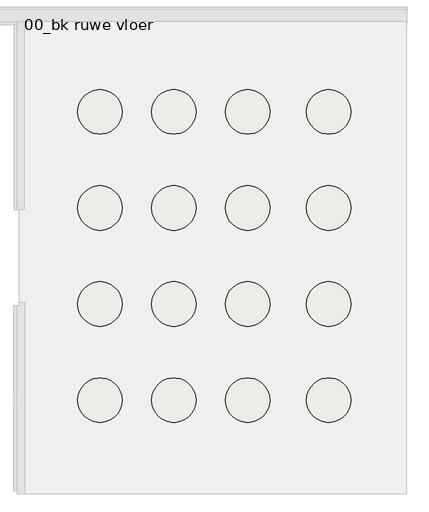
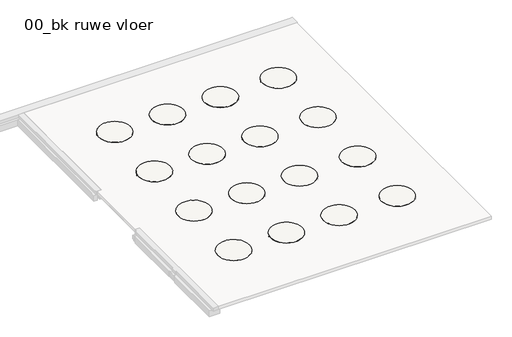
# One storey, part 3 of 6: 1 slab.
"""IFC4 building model written with IfcOpenShell, lengths in millimetres."""

from ifc_helpers import new_model, si_unit, frame, origin, place, context, project, spatial, circle_curve, element, save
from ifc_brep_helpers import plane_surface, cylinder_surface, advanced_brep

model = new_model("IFC4")

# Units and contexts
model_context = context("Model", 3, world=origin())
ifc_project = project(units=[si_unit("LENGTHUNIT", "METRE", prefix="MILLI")], contexts=[model_context])

# Site, building, storey
site = spatial("IfcSite", under=ifc_project)
building = spatial("IfcBuilding", under=site)
storey = spatial("IfcBuildingStorey", under=building, Name="00_bk ruwe vloer", Elevation=-70.0)

# Slab
placement = place(None, origin())
element("IfcSlab", 1, ObjectType="NLRS_23_FL_beton ihwg 450_gen_rsf", at=placement, inside=storey, context=model_context, shape_type="AdvancedBrep", body=[
    advanced_brep(
    [(34850.0, 37000.0, -520.0), (37850.0, 37000.0, -520.0), (37850.0, 37000.0, -70.0), (34850.0, 37000.0, -70.0), (34850.0, 37000.0, -390.0), (37850.0, 37000.0, -390.0), (37850.0, 37000.0, -330.0), (34850.0, 37000.0, -330.0), (37825.0, 37000.0, -390.0), (34875.0, 37000.0, -390.0), (37825.0, 37000.0, -330.0), (34875.0, 37000.0, -330.0)],
    [
        (0, 1, circle_curve(frame((36350.0, 37000.0, -520.0), z_axis=(0.0, 0.0, -1.0), x_axis=(1.0, 0.0, 0.0)), 1500.0)),
        (1, 0, circle_curve(frame((36350.0, 37000.0, -520.0), z_axis=(0.0, 0.0, -1.0), x_axis=(1.0, 0.0, 0.0)), 1500.0)),
        (2, 3, circle_curve(frame((36350.0, 37000.0, -70.0), z_axis=(0.0, 0.0, 1.0), x_axis=(1.0, 0.0, 0.0)), 1500.0)),
        (3, 2, circle_curve(frame((36350.0, 37000.0, -70.0), z_axis=(0.0, 0.0, 1.0), x_axis=(1.0, 0.0, 0.0)), 1500.0)),
        (0, 4),
        (4, 5, circle_curve(frame((36350.0, 37000.0, -390.0), z_axis=(0.0, 0.0, -1.0), x_axis=(1.0, 0.0, 0.0)), 1500.0)),
        (5, 1),
        (2, 6),
        (6, 7, circle_curve(frame((36350.0, 37000.0, -330.0), z_axis=(0.0, 0.0, 1.0), x_axis=(1.0, 0.0, 0.0)), 1500.0)),
        (7, 3),
        (5, 4, circle_curve(frame((36350.0, 37000.0, -390.0), z_axis=(0.0, 0.0, -1.0), x_axis=(1.0, 0.0, 0.0)), 1500.0)),
        (7, 6, circle_curve(frame((36350.0, 37000.0, -330.0), z_axis=(0.0, 0.0, 1.0), x_axis=(1.0, 0.0, 0.0)), 1500.0)),
        (8, 9, circle_curve(frame((36350.0, 37000.0, -390.0), z_axis=(0.0, 0.0, -1.0), x_axis=(1.0, 0.0, 0.0)), 1475.0)),
        (9, 8, circle_curve(frame((36350.0, 37000.0, -390.0), z_axis=(0.0, 0.0, -1.0), x_axis=(1.0, 0.0, 0.0)), 1475.0)),
        (10, 11, circle_curve(frame((36350.0, 37000.0, -330.0), z_axis=(0.0, 0.0, 1.0), x_axis=(1.0, 0.0, 0.0)), 1475.0)),
        (11, 10, circle_curve(frame((36350.0, 37000.0, -330.0), z_axis=(0.0, 0.0, 1.0), x_axis=(1.0, 0.0, 0.0)), 1475.0)),
        (8, 10),
        (11, 9),
    ],
    [
        plane_surface(frame((37850.0, 37000.0, -520.0), z_axis=(0.0, 0.0, -1.0), x_axis=(0.0, -1.0, 0.0))),
        plane_surface(frame((37850.0, 37000.0, -70.0), z_axis=(0.0, 0.0, 1.0), x_axis=(0.0, 1.0, 0.0))),
        cylinder_surface(frame((36350.0, 37000.0, -70.0), z_axis=(0.0, 0.0, -1.0), x_axis=(1.0, 0.0, 0.0)), 1500.0),
        plane_surface(frame((51875.0, 42925.0, -390.0), z_axis=(0.0, 0.0, 1.0), x_axis=(1.0, 0.0, 0.0))),
        plane_surface(frame((51875.0, 42925.0, -330.0), z_axis=(0.0, 0.0, -1.0), x_axis=(-1.0, 0.0, 0.0))),
        cylinder_surface(frame((36350.0, 37000.0, -70.0), z_axis=(0.0, 0.0, 1.0), x_axis=(1.0, 0.0, 0.0)), 1475.0),
    ],
    [
        (0, [[1, 2]]),
        (1, [[3, 4]]),
        (2, [[-1, 5, 6, 7]]),
        (2, [[-3, 8, 9, 10]]),
        (2, [[-2, -7, 11, -5]]),
        (2, [[-4, -10, 12, -8]]),
        (3, [[-6, -11], [13, 14]]),
        (4, [[-9, -12], [15, 16]]),
        (5, [[-13, 17, -16, 18]]),
        (5, [[-14, -18, -15, -17]]),
    ],
),
    advanced_brep(
    [(45350.0, 37000.0, -520.0), (48350.0, 37000.0, -520.0), (48350.0, 37000.0, -70.0), (45350.0, 37000.0, -70.0), (45350.0, 37000.0, -390.0), (48350.0, 37000.0, -390.0), (48350.0, 37000.0, -330.0), (45350.0, 37000.0, -330.0), (48325.0, 37000.0, -390.0), (45375.0, 37000.0, -390.0), (48325.0, 37000.0, -330.0), (45375.0, 37000.0, -330.0)],
    [
        (0, 1, circle_curve(frame((46850.0, 37000.0, -520.0), z_axis=(0.0, 0.0, -1.0), x_axis=(1.0, 0.0, 0.0)), 1500.0)),
        (1, 0, circle_curve(frame((46850.0, 37000.0, -520.0), z_axis=(0.0, 0.0, -1.0), x_axis=(1.0, 0.0, 0.0)), 1500.0)),
        (2, 3, circle_curve(frame((46850.0, 37000.0, -70.0), z_axis=(0.0, 0.0, 1.0), x_axis=(1.0, 0.0, 0.0)), 1500.0)),
        (3, 2, circle_curve(frame((46850.0, 37000.0, -70.0), z_axis=(0.0, 0.0, 1.0), x_axis=(1.0, 0.0, 0.0)), 1500.0)),
        (0, 4),
        (4, 5, circle_curve(frame((46850.0, 37000.0, -390.0), z_axis=(0.0, 0.0, -1.0), x_axis=(1.0, 0.0, 0.0)), 1500.0)),
        (5, 1),
        (2, 6),
        (6, 7, circle_curve(frame((46850.0, 37000.0, -330.0), z_axis=(0.0, 0.0, 1.0), x_axis=(1.0, 0.0, 0.0)), 1500.0)),
        (7, 3),
        (5, 4, circle_curve(frame((46850.0, 37000.0, -390.0), z_axis=(0.0, 0.0, -1.0), x_axis=(1.0, 0.0, 0.0)), 1500.0)),
        (7, 6, circle_curve(frame((46850.0, 37000.0, -330.0), z_axis=(0.0, 0.0, 1.0), x_axis=(1.0, 0.0, 0.0)), 1500.0)),
        (8, 9, circle_curve(frame((46850.0, 37000.0, -390.0), z_axis=(0.0, 0.0, -1.0), x_axis=(1.0, 0.0, 0.0)), 1475.0)),
        (9, 8, circle_curve(frame((46850.0, 37000.0, -390.0), z_axis=(0.0, 0.0, -1.0), x_axis=(1.0, 0.0, 0.0)), 1475.0)),
        (10, 11, circle_curve(frame((46850.0, 37000.0, -330.0), z_axis=(0.0, 0.0, 1.0), x_axis=(1.0, 0.0, 0.0)), 1475.0)),
        (11, 10, circle_curve(frame((46850.0, 37000.0, -330.0), z_axis=(0.0, 0.0, 1.0), x_axis=(1.0, 0.0, 0.0)), 1475.0)),
        (8, 10),
        (11, 9),
    ],
    [
        plane_surface(frame((37850.0, 37000.0, -520.0), z_axis=(0.0, 0.0, -1.0), x_axis=(0.0, -1.0, 0.0))),
        plane_surface(frame((37850.0, 37000.0, -70.0), z_axis=(0.0, 0.0, 1.0), x_axis=(0.0, 1.0, 0.0))),
        cylinder_surface(frame((46850.0, 37000.0, -70.0), z_axis=(0.0, 0.0, -1.0), x_axis=(1.0, 0.0, 0.0)), 1500.0),
        plane_surface(frame((51875.0, 42925.0, -390.0), z_axis=(0.0, 0.0, 1.0), x_axis=(1.0, 0.0, 0.0))),
        plane_surface(frame((51875.0, 42925.0, -330.0), z_axis=(0.0, 0.0, -1.0), x_axis=(-1.0, 0.0, 0.0))),
        cylinder_surface(frame((46850.0, 37000.0, -70.0), z_axis=(0.0, 0.0, 1.0), x_axis=(1.0, 0.0, 0.0)), 1475.0),
    ],
    [
        (0, [[1, 2]]),
        (1, [[3, 4]]),
        (2, [[-1, 5, 6, 7]]),
        (2, [[-3, 8, 9, 10]]),
        (2, [[-2, -7, 11, -5]]),
        (2, [[-4, -10, 12, -8]]),
        (3, [[-6, -11], [13, 14]]),
        (4, [[-9, -12], [15, 16]]),
        (5, [[-13, 17, -16, 18]]),
        (5, [[-14, -18, -15, -17]]),
    ],
),
    advanced_brep(
    [(45350.0, 30500.0, -520.0), (48350.0, 30500.0, -520.0), (48350.0, 30500.0, -70.0), (45350.0, 30500.0, -70.0), (45350.0, 30500.0, -390.0), (48350.0, 30500.0, -390.0), (48350.0, 30500.0, -330.0), (45350.0, 30500.0, -330.0), (48325.0, 30500.0, -390.0), (45375.0, 30500.0, -390.0), (48325.0, 30500.0, -330.0), (45375.0, 30500.0, -330.0)],
    [
        (0, 1, circle_curve(frame((46850.0, 30500.0, -520.0), z_axis=(0.0, 0.0, -1.0), x_axis=(1.0, 0.0, 0.0)), 1500.0)),
        (1, 0, circle_curve(frame((46850.0, 30500.0, -520.0), z_axis=(0.0, 0.0, -1.0), x_axis=(1.0, 0.0, 0.0)), 1500.0)),
        (2, 3, circle_curve(frame((46850.0, 30500.0, -70.0), z_axis=(0.0, 0.0, 1.0), x_axis=(1.0, 0.0, 0.0)), 1500.0)),
        (3, 2, circle_curve(frame((46850.0, 30500.0, -70.0), z_axis=(0.0, 0.0, 1.0), x_axis=(1.0, 0.0, 0.0)), 1500.0)),
        (0, 4),
        (4, 5, circle_curve(frame((46850.0, 30500.0, -390.0), z_axis=(0.0, 0.0, -1.0), x_axis=(1.0, 0.0, 0.0)), 1500.0)),
        (5, 1),
        (2, 6),
        (6, 7, circle_curve(frame((46850.0, 30500.0, -330.0), z_axis=(0.0, 0.0, 1.0), x_axis=(1.0, 0.0, 0.0)), 1500.0)),
        (7, 3),
        (5, 4, circle_curve(frame((46850.0, 30500.0, -390.0), z_axis=(0.0, 0.0, -1.0), x_axis=(1.0, 0.0, 0.0)), 1500.0)),
        (7, 6, circle_curve(frame((46850.0, 30500.0, -330.0), z_axis=(0.0, 0.0, 1.0), x_axis=(1.0, 0.0, 0.0)), 1500.0)),
        (8, 9, circle_curve(frame((46850.0, 30500.0, -390.0), z_axis=(0.0, 0.0, -1.0), x_axis=(1.0, 0.0, 0.0)), 1475.0)),
        (9, 8, circle_curve(frame((46850.0, 30500.0, -390.0), z_axis=(0.0, 0.0, -1.0), x_axis=(1.0, 0.0, 0.0)), 1475.0)),
        (10, 11, circle_curve(frame((46850.0, 30500.0, -330.0), z_axis=(0.0, 0.0, 1.0), x_axis=(1.0, 0.0, 0.0)), 1475.0)),
        (11, 10, circle_curve(frame((46850.0, 30500.0, -330.0), z_axis=(0.0, 0.0, 1.0), x_axis=(1.0, 0.0, 0.0)), 1475.0)),
        (8, 10),
        (11, 9),
    ],
    [
        plane_surface(frame((37850.0, 37000.0, -520.0), z_axis=(0.0, 0.0, -1.0), x_axis=(0.0, -1.0, 0.0))),
        plane_surface(frame((37850.0, 37000.0, -70.0), z_axis=(0.0, 0.0, 1.0), x_axis=(0.0, 1.0, 0.0))),
        cylinder_surface(frame((46850.0, 30500.0, -70.0), z_axis=(0.0, 0.0, -1.0), x_axis=(1.0, 0.0, 0.0)), 1500.0),
        plane_surface(frame((51875.0, 42925.0, -390.0), z_axis=(0.0, 0.0, 1.0), x_axis=(1.0, 0.0, 0.0))),
        plane_surface(frame((51875.0, 42925.0, -330.0), z_axis=(0.0, 0.0, -1.0), x_axis=(-1.0, 0.0, 0.0))),
        cylinder_surface(frame((46850.0, 30500.0, -70.0), z_axis=(0.0, 0.0, 1.0), x_axis=(1.0, 0.0, 0.0)), 1475.0),
    ],
    [
        (0, [[1, 2]]),
        (1, [[3, 4]]),
        (2, [[-1, 5, 6, 7]]),
        (2, [[-3, 8, 9, 10]]),
        (2, [[-2, -7, 11, -5]]),
        (2, [[-4, -10, 12, -8]]),
        (3, [[-6, -11], [13, 14]]),
        (4, [[-9, -12], [15, 16]]),
        (5, [[-13, 17, -16, 18]]),
        (5, [[-14, -18, -15, -17]]),
    ],
),
    advanced_brep(
    [(34850.0, 30500.0, -520.0), (37850.0, 30500.0, -520.0), (37850.0, 30500.0, -70.0), (34850.0, 30500.0, -70.0), (34850.0, 30500.0, -390.0), (37850.0, 30500.0, -390.0), (37850.0, 30500.0, -330.0), (34850.0, 30500.0, -330.0), (37825.0, 30500.0, -390.0), (34875.0, 30500.0, -390.0), (37825.0, 30500.0, -330.0), (34875.0, 30500.0, -330.0)],
    [
        (0, 1, circle_curve(frame((36350.0, 30500.0, -520.0), z_axis=(0.0, 0.0, -1.0), x_axis=(1.0, 0.0, 0.0)), 1500.0)),
        (1, 0, circle_curve(frame((36350.0, 30500.0, -520.0), z_axis=(0.0, 0.0, -1.0), x_axis=(1.0, 0.0, 0.0)), 1500.0)),
        (2, 3, circle_curve(frame((36350.0, 30500.0, -70.0), z_axis=(0.0, 0.0, 1.0), x_axis=(1.0, 0.0, 0.0)), 1500.0)),
        (3, 2, circle_curve(frame((36350.0, 30500.0, -70.0), z_axis=(0.0, 0.0, 1.0), x_axis=(1.0, 0.0, 0.0)), 1500.0)),
        (0, 4),
        (4, 5, circle_curve(frame((36350.0, 30500.0, -390.0), z_axis=(0.0, 0.0, -1.0), x_axis=(1.0, 0.0, 0.0)), 1500.0)),
        (5, 1),
        (2, 6),
        (6, 7, circle_curve(frame((36350.0, 30500.0, -330.0), z_axis=(0.0, 0.0, 1.0), x_axis=(1.0, 0.0, 0.0)), 1500.0)),
        (7, 3),
        (5, 4, circle_curve(frame((36350.0, 30500.0, -390.0), z_axis=(0.0, 0.0, -1.0), x_axis=(1.0, 0.0, 0.0)), 1500.0)),
        (7, 6, circle_curve(frame((36350.0, 30500.0, -330.0), z_axis=(0.0, 0.0, 1.0), x_axis=(1.0, 0.0, 0.0)), 1500.0)),
        (8, 9, circle_curve(frame((36350.0, 30500.0, -390.0), z_axis=(0.0, 0.0, -1.0), x_axis=(1.0, 0.0, 0.0)), 1475.0)),
        (9, 8, circle_curve(frame((36350.0, 30500.0, -390.0), z_axis=(0.0, 0.0, -1.0), x_axis=(1.0, 0.0, 0.0)), 1475.0)),
        (10, 11, circle_curve(frame((36350.0, 30500.0, -330.0), z_axis=(0.0, 0.0, 1.0), x_axis=(1.0, 0.0, 0.0)), 1475.0)),
        (11, 10, circle_curve(frame((36350.0, 30500.0, -330.0), z_axis=(0.0, 0.0, 1.0), x_axis=(1.0, 0.0, 0.0)), 1475.0)),
        (8, 10),
        (11, 9),
    ],
    [
        plane_surface(frame((37850.0, 37000.0, -520.0), z_axis=(0.0, 0.0, -1.0), x_axis=(0.0, -1.0, 0.0))),
        plane_surface(frame((37850.0, 37000.0, -70.0), z_axis=(0.0, 0.0, 1.0), x_axis=(0.0, 1.0, 0.0))),
        cylinder_surface(frame((36350.0, 30500.0, -70.0), z_axis=(0.0, 0.0, -1.0), x_axis=(1.0, 0.0, 0.0)), 1500.0),
        plane_surface(frame((51875.0, 42925.0, -390.0), z_axis=(0.0, 0.0, 1.0), x_axis=(1.0, 0.0, 0.0))),
        plane_surface(frame((51875.0, 42925.0, -330.0), z_axis=(0.0, 0.0, -1.0), x_axis=(-1.0, 0.0, 0.0))),
        cylinder_surface(frame((36350.0, 30500.0, -70.0), z_axis=(0.0, 0.0, 1.0), x_axis=(1.0, 0.0, 0.0)), 1475.0),
    ],
    [
        (0, [[1, 2]]),
        (1, [[3, 4]]),
        (2, [[-1, 5, 6, 7]]),
        (2, [[-3, 8, 9, 10]]),
        (2, [[-2, -7, 11, -5]]),
        (2, [[-4, -10, 12, -8]]),
        (3, [[-6, -11], [13, 14]]),
        (4, [[-9, -12], [15, 16]]),
        (5, [[-13, 17, -16, 18]]),
        (5, [[-14, -18, -15, -17]]),
    ],
),
    advanced_brep(
    [(34850.0, 24000.0, -520.0), (37850.0, 24000.0, -520.0), (37850.0, 24000.0, -70.0), (34850.0, 24000.0, -70.0), (34850.0, 24000.0, -390.0), (37850.0, 24000.0, -390.0), (37850.0, 24000.0, -330.0), (34850.0, 24000.0, -330.0), (37825.0, 24000.0, -390.0), (34875.0, 24000.0, -390.0), (37825.0, 24000.0, -330.0), (34875.0, 24000.0, -330.0)],
    [
        (0, 1, circle_curve(frame((36350.0, 24000.0, -520.0), z_axis=(0.0, 0.0, -1.0), x_axis=(1.0, 0.0, 0.0)), 1500.0)),
        (1, 0, circle_curve(frame((36350.0, 24000.0, -520.0), z_axis=(0.0, 0.0, -1.0), x_axis=(1.0, 0.0, 0.0)), 1500.0)),
        (2, 3, circle_curve(frame((36350.0, 24000.0, -70.0), z_axis=(0.0, 0.0, 1.0), x_axis=(1.0, 0.0, 0.0)), 1500.0)),
        (3, 2, circle_curve(frame((36350.0, 24000.0, -70.0), z_axis=(0.0, 0.0, 1.0), x_axis=(1.0, 0.0, 0.0)), 1500.0)),
        (0, 4),
        (4, 5, circle_curve(frame((36350.0, 24000.0, -390.0), z_axis=(0.0, 0.0, -1.0), x_axis=(1.0, 0.0, 0.0)), 1500.0)),
        (5, 1),
        (2, 6),
        (6, 7, circle_curve(frame((36350.0, 24000.0, -330.0), z_axis=(0.0, 0.0, 1.0), x_axis=(1.0, 0.0, 0.0)), 1500.0)),
        (7, 3),
        (5, 4, circle_curve(frame((36350.0, 24000.0, -390.0), z_axis=(0.0, 0.0, -1.0), x_axis=(1.0, 0.0, 0.0)), 1500.0)),
        (7, 6, circle_curve(frame((36350.0, 24000.0, -330.0), z_axis=(0.0, 0.0, 1.0), x_axis=(1.0, 0.0, 0.0)), 1500.0)),
        (8, 9, circle_curve(frame((36350.0, 24000.0, -390.0), z_axis=(0.0, 0.0, -1.0), x_axis=(1.0, 0.0, 0.0)), 1475.0)),
        (9, 8, circle_curve(frame((36350.0, 24000.0, -390.0), z_axis=(0.0, 0.0, -1.0), x_axis=(1.0, 0.0, 0.0)), 1475.0)),
        (10, 11, circle_curve(frame((36350.0, 24000.0, -330.0), z_axis=(0.0, 0.0, 1.0), x_axis=(1.0, 0.0, 0.0)), 1475.0)),
        (11, 10, circle_curve(frame((36350.0, 24000.0, -330.0), z_axis=(0.0, 0.0, 1.0), x_axis=(1.0, 0.0, 0.0)), 1475.0)),
        (8, 10),
        (11, 9),
    ],
    [
        plane_surface(frame((37850.0, 37000.0, -520.0), z_axis=(0.0, 0.0, -1.0), x_axis=(0.0, -1.0, 0.0))),
        plane_surface(frame((37850.0, 37000.0, -70.0), z_axis=(0.0, 0.0, 1.0), x_axis=(0.0, 1.0, 0.0))),
        cylinder_surface(frame((36350.0, 24000.0, -70.0), z_axis=(0.0, 0.0, -1.0), x_axis=(1.0, 0.0, 0.0)), 1500.0),
        plane_surface(frame((51875.0, 42925.0, -390.0), z_axis=(0.0, 0.0, 1.0), x_axis=(1.0, 0.0, 0.0))),
        plane_surface(frame((51875.0, 42925.0, -330.0), z_axis=(0.0, 0.0, -1.0), x_axis=(-1.0, 0.0, 0.0))),
        cylinder_surface(frame((36350.0, 24000.0, -70.0), z_axis=(0.0, 0.0, 1.0), x_axis=(1.0, 0.0, 0.0)), 1475.0),
    ],
    [
        (0, [[1, 2]]),
        (1, [[3, 4]]),
        (2, [[-1, 5, 6, 7]]),
        (2, [[-3, 8, 9, 10]]),
        (2, [[-2, -7, 11, -5]]),
        (2, [[-4, -10, 12, -8]]),
        (3, [[-6, -11], [13, 14]]),
        (4, [[-9, -12], [15, 16]]),
        (5, [[-13, 17, -16, 18]]),
        (5, [[-14, -18, -15, -17]]),
    ],
),
    advanced_brep(
    [(45350.0, 24000.0, -520.0), (48350.0, 24000.0, -520.0), (48350.0, 24000.0, -70.0), (45350.0, 24000.0, -70.0), (45350.0, 24000.0, -390.0), (48350.0, 24000.0, -390.0), (48350.0, 24000.0, -330.0), (45350.0, 24000.0, -330.0), (48325.0, 24000.0, -390.0), (45375.0, 24000.0, -390.0), (48325.0, 24000.0, -330.0), (45375.0, 24000.0, -330.0)],
    [
        (0, 1, circle_curve(frame((46850.0, 24000.0, -520.0), z_axis=(0.0, 0.0, -1.0), x_axis=(1.0, 0.0, 0.0)), 1500.0)),
        (1, 0, circle_curve(frame((46850.0, 24000.0, -520.0), z_axis=(0.0, 0.0, -1.0), x_axis=(1.0, 0.0, 0.0)), 1500.0)),
        (2, 3, circle_curve(frame((46850.0, 24000.0, -70.0), z_axis=(0.0, 0.0, 1.0), x_axis=(1.0, 0.0, 0.0)), 1500.0)),
        (3, 2, circle_curve(frame((46850.0, 24000.0, -70.0), z_axis=(0.0, 0.0, 1.0), x_axis=(1.0, 0.0, 0.0)), 1500.0)),
        (0, 4),
        (4, 5, circle_curve(frame((46850.0, 24000.0, -390.0), z_axis=(0.0, 0.0, -1.0), x_axis=(1.0, 0.0, 0.0)), 1500.0)),
        (5, 1),
        (2, 6),
        (6, 7, circle_curve(frame((46850.0, 24000.0, -330.0), z_axis=(0.0, 0.0, 1.0), x_axis=(1.0, 0.0, 0.0)), 1500.0)),
        (7, 3),
        (5, 4, circle_curve(frame((46850.0, 24000.0, -390.0), z_axis=(0.0, 0.0, -1.0), x_axis=(1.0, 0.0, 0.0)), 1500.0)),
        (7, 6, circle_curve(frame((46850.0, 24000.0, -330.0), z_axis=(0.0, 0.0, 1.0), x_axis=(1.0, 0.0, 0.0)), 1500.0)),
        (8, 9, circle_curve(frame((46850.0, 24000.0, -390.0), z_axis=(0.0, 0.0, -1.0), x_axis=(1.0, 0.0, 0.0)), 1475.0)),
        (9, 8, circle_curve(frame((46850.0, 24000.0, -390.0), z_axis=(0.0, 0.0, -1.0), x_axis=(1.0, 0.0, 0.0)), 1475.0)),
        (10, 11, circle_curve(frame((46850.0, 24000.0, -330.0), z_axis=(0.0, 0.0, 1.0), x_axis=(1.0, 0.0, 0.0)), 1475.0)),
        (11, 10, circle_curve(frame((46850.0, 24000.0, -330.0), z_axis=(0.0, 0.0, 1.0), x_axis=(1.0, 0.0, 0.0)), 1475.0)),
        (8, 10),
        (11, 9),
    ],
    [
        plane_surface(frame((37850.0, 37000.0, -520.0), z_axis=(0.0, 0.0, -1.0), x_axis=(0.0, -1.0, 0.0))),
        plane_surface(frame((37850.0, 37000.0, -70.0), z_axis=(0.0, 0.0, 1.0), x_axis=(0.0, 1.0, 0.0))),
        cylinder_surface(frame((46850.0, 24000.0, -70.0), z_axis=(0.0, 0.0, -1.0), x_axis=(1.0, 0.0, 0.0)), 1500.0),
        plane_surface(frame((51875.0, 42925.0, -390.0), z_axis=(0.0, 0.0, 1.0), x_axis=(1.0, 0.0, 0.0))),
        plane_surface(frame((51875.0, 42925.0, -330.0), z_axis=(0.0, 0.0, -1.0), x_axis=(-1.0, 0.0, 0.0))),
        cylinder_surface(frame((46850.0, 24000.0, -70.0), z_axis=(0.0, 0.0, 1.0), x_axis=(1.0, 0.0, 0.0)), 1475.0),
    ],
    [
        (0, [[1, 2]]),
        (1, [[3, 4]]),
        (2, [[-1, 5, 6, 7]]),
        (2, [[-3, 8, 9, 10]]),
        (2, [[-2, -7, 11, -5]]),
        (2, [[-4, -10, 12, -8]]),
        (3, [[-6, -11], [13, 14]]),
        (4, [[-9, -12], [15, 16]]),
        (5, [[-13, 17, -16, 18]]),
        (5, [[-14, -18, -15, -17]]),
    ],
),
    advanced_brep(
    [(45350.0, 17500.0, -520.0), (48350.0, 17500.0, -520.0), (48350.0, 17500.0, -70.0), (45350.0, 17500.0, -70.0), (45350.0, 17500.0, -390.0), (48350.0, 17500.0, -390.0), (48350.0, 17500.0, -330.0), (45350.0, 17500.0, -330.0), (48325.0, 17500.0, -390.0), (45375.0, 17500.0, -390.0), (48325.0, 17500.0, -330.0), (45375.0, 17500.0, -330.0)],
    [
        (0, 1, circle_curve(frame((46850.0, 17500.0, -520.0), z_axis=(0.0, 0.0, -1.0), x_axis=(1.0, 0.0, 0.0)), 1500.0)),
        (1, 0, circle_curve(frame((46850.0, 17500.0, -520.0), z_axis=(0.0, 0.0, -1.0), x_axis=(1.0, 0.0, 0.0)), 1500.0)),
        (2, 3, circle_curve(frame((46850.0, 17500.0, -70.0), z_axis=(0.0, 0.0, 1.0), x_axis=(1.0, 0.0, 0.0)), 1500.0)),
        (3, 2, circle_curve(frame((46850.0, 17500.0, -70.0), z_axis=(0.0, 0.0, 1.0), x_axis=(1.0, 0.0, 0.0)), 1500.0)),
        (0, 4),
        (4, 5, circle_curve(frame((46850.0, 17500.0, -390.0), z_axis=(0.0, 0.0, -1.0), x_axis=(1.0, 0.0, 0.0)), 1500.0)),
        (5, 1),
        (2, 6),
        (6, 7, circle_curve(frame((46850.0, 17500.0, -330.0), z_axis=(0.0, 0.0, 1.0), x_axis=(1.0, 0.0, 0.0)), 1500.0)),
        (7, 3),
        (5, 4, circle_curve(frame((46850.0, 17500.0, -390.0), z_axis=(0.0, 0.0, -1.0), x_axis=(1.0, 0.0, 0.0)), 1500.0)),
        (7, 6, circle_curve(frame((46850.0, 17500.0, -330.0), z_axis=(0.0, 0.0, 1.0), x_axis=(1.0, 0.0, 0.0)), 1500.0)),
        (8, 9, circle_curve(frame((46850.0, 17500.0, -390.0), z_axis=(0.0, 0.0, -1.0), x_axis=(1.0, 0.0, 0.0)), 1475.0)),
        (9, 8, circle_curve(frame((46850.0, 17500.0, -390.0), z_axis=(0.0, 0.0, -1.0), x_axis=(1.0, 0.0, 0.0)), 1475.0)),
        (10, 11, circle_curve(frame((46850.0, 17500.0, -330.0), z_axis=(0.0, 0.0, 1.0), x_axis=(1.0, 0.0, 0.0)), 1475.0)),
        (11, 10, circle_curve(frame((46850.0, 17500.0, -330.0), z_axis=(0.0, 0.0, 1.0), x_axis=(1.0, 0.0, 0.0)), 1475.0)),
        (8, 10),
        (11, 9),
    ],
    [
        plane_surface(frame((37850.0, 37000.0, -520.0), z_axis=(0.0, 0.0, -1.0), x_axis=(0.0, -1.0, 0.0))),
        plane_surface(frame((37850.0, 37000.0, -70.0), z_axis=(0.0, 0.0, 1.0), x_axis=(0.0, 1.0, 0.0))),
        cylinder_surface(frame((46850.0, 17500.0, -70.0), z_axis=(0.0, 0.0, -1.0), x_axis=(1.0, 0.0, 0.0)), 1500.0),
        plane_surface(frame((51875.0, 42925.0, -390.0), z_axis=(0.0, 0.0, 1.0), x_axis=(1.0, 0.0, 0.0))),
        plane_surface(frame((51875.0, 42925.0, -330.0), z_axis=(0.0, 0.0, -1.0), x_axis=(-1.0, 0.0, 0.0))),
        cylinder_surface(frame((46850.0, 17500.0, -70.0), z_axis=(0.0, 0.0, 1.0), x_axis=(1.0, 0.0, 0.0)), 1475.0),
    ],
    [
        (0, [[1, 2]]),
        (1, [[3, 4]]),
        (2, [[-1, 5, 6, 7]]),
        (2, [[-3, 8, 9, 10]]),
        (2, [[-2, -7, 11, -5]]),
        (2, [[-4, -10, 12, -8]]),
        (3, [[-6, -11], [13, 14]]),
        (4, [[-9, -12], [15, 16]]),
        (5, [[-13, 17, -16, 18]]),
        (5, [[-14, -18, -15, -17]]),
    ],
),
    advanced_brep(
    [(34850.0, 17500.0, -520.0), (37850.0, 17500.0, -520.0), (37850.0, 17500.0, -70.0), (34850.0, 17500.0, -70.0), (34850.0, 17500.0, -390.0), (37850.0, 17500.0, -390.0), (37850.0, 17500.0, -330.0), (34850.0, 17500.0, -330.0), (37825.0, 17500.0, -390.0), (34875.0, 17500.0, -390.0), (37825.0, 17500.0, -330.0), (34875.0, 17500.0, -330.0)],
    [
        (0, 1, circle_curve(frame((36350.0, 17500.0, -520.0), z_axis=(0.0, 0.0, -1.0), x_axis=(1.0, 0.0, 0.0)), 1500.0)),
        (1, 0, circle_curve(frame((36350.0, 17500.0, -520.0), z_axis=(0.0, 0.0, -1.0), x_axis=(1.0, 0.0, 0.0)), 1500.0)),
        (2, 3, circle_curve(frame((36350.0, 17500.0, -70.0), z_axis=(0.0, 0.0, 1.0), x_axis=(1.0, 0.0, 0.0)), 1500.0)),
        (3, 2, circle_curve(frame((36350.0, 17500.0, -70.0), z_axis=(0.0, 0.0, 1.0), x_axis=(1.0, 0.0, 0.0)), 1500.0)),
        (0, 4),
        (4, 5, circle_curve(frame((36350.0, 17500.0, -390.0), z_axis=(0.0, 0.0, -1.0), x_axis=(1.0, 0.0, 0.0)), 1500.0)),
        (5, 1),
        (2, 6),
        (6, 7, circle_curve(frame((36350.0, 17500.0, -330.0), z_axis=(0.0, 0.0, 1.0), x_axis=(1.0, 0.0, 0.0)), 1500.0)),
        (7, 3),
        (5, 4, circle_curve(frame((36350.0, 17500.0, -390.0), z_axis=(0.0, 0.0, -1.0), x_axis=(1.0, 0.0, 0.0)), 1500.0)),
        (7, 6, circle_curve(frame((36350.0, 17500.0, -330.0), z_axis=(0.0, 0.0, 1.0), x_axis=(1.0, 0.0, 0.0)), 1500.0)),
        (8, 9, circle_curve(frame((36350.0, 17500.0, -390.0), z_axis=(0.0, 0.0, -1.0), x_axis=(1.0, 0.0, 0.0)), 1475.0)),
        (9, 8, circle_curve(frame((36350.0, 17500.0, -390.0), z_axis=(0.0, 0.0, -1.0), x_axis=(1.0, 0.0, 0.0)), 1475.0)),
        (10, 11, circle_curve(frame((36350.0, 17500.0, -330.0), z_axis=(0.0, 0.0, 1.0), x_axis=(1.0, 0.0, 0.0)), 1475.0)),
        (11, 10, circle_curve(frame((36350.0, 17500.0, -330.0), z_axis=(0.0, 0.0, 1.0), x_axis=(1.0, 0.0, 0.0)), 1475.0)),
        (8, 10),
        (11, 9),
    ],
    [
        plane_surface(frame((37850.0, 37000.0, -520.0), z_axis=(0.0, 0.0, -1.0), x_axis=(0.0, -1.0, 0.0))),
        plane_surface(frame((37850.0, 37000.0, -70.0), z_axis=(0.0, 0.0, 1.0), x_axis=(0.0, 1.0, 0.0))),
        cylinder_surface(frame((36350.0, 17500.0, -70.0), z_axis=(0.0, 0.0, -1.0), x_axis=(1.0, 0.0, 0.0)), 1500.0),
        plane_surface(frame((51875.0, 42925.0, -390.0), z_axis=(0.0, 0.0, 1.0), x_axis=(1.0, 0.0, 0.0))),
        plane_surface(frame((51875.0, 42925.0, -330.0), z_axis=(0.0, 0.0, -1.0), x_axis=(-1.0, 0.0, 0.0))),
        cylinder_surface(frame((36350.0, 17500.0, -70.0), z_axis=(0.0, 0.0, 1.0), x_axis=(1.0, 0.0, 0.0)), 1475.0),
    ],
    [
        (0, [[1, 2]]),
        (1, [[3, 4]]),
        (2, [[-1, 5, 6, 7]]),
        (2, [[-3, 8, 9, 10]]),
        (2, [[-2, -7, 11, -5]]),
        (2, [[-4, -10, 12, -8]]),
        (3, [[-6, -11], [13, 14]]),
        (4, [[-9, -12], [15, 16]]),
        (5, [[-13, 17, -16, 18]]),
        (5, [[-14, -18, -15, -17]]),
    ],
),
    advanced_brep(
    [(39850.0, 37000.0, -520.0), (42850.0, 37000.0, -520.0), (42850.0, 37000.0, -70.0), (39850.0, 37000.0, -70.0), (39850.0, 37000.0, -390.0), (42850.0, 37000.0, -390.0), (42850.0, 37000.0, -330.0), (39850.0, 37000.0, -330.0), (42825.0, 37000.0, -390.0), (39875.0, 37000.0, -390.0), (42825.0, 37000.0, -330.0), (39875.0, 37000.0, -330.0)],
    [
        (0, 1, circle_curve(frame((41350.0, 37000.0, -520.0), z_axis=(0.0, 0.0, -1.0), x_axis=(1.0, 0.0, 0.0)), 1500.0)),
        (1, 0, circle_curve(frame((41350.0, 37000.0, -520.0), z_axis=(0.0, 0.0, -1.0), x_axis=(1.0, 0.0, 0.0)), 1500.0)),
        (2, 3, circle_curve(frame((41350.0, 37000.0, -70.0), z_axis=(0.0, 0.0, 1.0), x_axis=(1.0, 0.0, 0.0)), 1500.0)),
        (3, 2, circle_curve(frame((41350.0, 37000.0, -70.0), z_axis=(0.0, 0.0, 1.0), x_axis=(1.0, 0.0, 0.0)), 1500.0)),
        (0, 4),
        (4, 5, circle_curve(frame((41350.0, 37000.0, -390.0), z_axis=(0.0, 0.0, -1.0), x_axis=(1.0, 0.0, 0.0)), 1500.0)),
        (5, 1),
        (2, 6),
        (6, 7, circle_curve(frame((41350.0, 37000.0, -330.0), z_axis=(0.0, 0.0, 1.0), x_axis=(1.0, 0.0, 0.0)), 1500.0)),
        (7, 3),
        (5, 4, circle_curve(frame((41350.0, 37000.0, -390.0), z_axis=(0.0, 0.0, -1.0), x_axis=(1.0, 0.0, 0.0)), 1500.0)),
        (7, 6, circle_curve(frame((41350.0, 37000.0, -330.0), z_axis=(0.0, 0.0, 1.0), x_axis=(1.0, 0.0, 0.0)), 1500.0)),
        (8, 9, circle_curve(frame((41350.0, 37000.0, -390.0), z_axis=(0.0, 0.0, -1.0), x_axis=(1.0, 0.0, 0.0)), 1475.0)),
        (9, 8, circle_curve(frame((41350.0, 37000.0, -390.0), z_axis=(0.0, 0.0, -1.0), x_axis=(1.0, 0.0, 0.0)), 1475.0)),
        (10, 11, circle_curve(frame((41350.0, 37000.0, -330.0), z_axis=(0.0, 0.0, 1.0), x_axis=(1.0, 0.0, 0.0)), 1475.0)),
        (11, 10, circle_curve(frame((41350.0, 37000.0, -330.0), z_axis=(0.0, 0.0, 1.0), x_axis=(1.0, 0.0, 0.0)), 1475.0)),
        (8, 10),
        (11, 9),
    ],
    [
        plane_surface(frame((37850.0, 37000.0, -520.0), z_axis=(0.0, 0.0, -1.0), x_axis=(0.0, -1.0, 0.0))),
        plane_surface(frame((37850.0, 37000.0, -70.0), z_axis=(0.0, 0.0, 1.0), x_axis=(0.0, 1.0, 0.0))),
        cylinder_surface(frame((41350.0, 37000.0, -70.0), z_axis=(0.0, 0.0, -1.0), x_axis=(1.0, 0.0, 0.0)), 1500.0),
        plane_surface(frame((51875.0, 42925.0, -390.0), z_axis=(0.0, 0.0, 1.0), x_axis=(1.0, 0.0, 0.0))),
        plane_surface(frame((51875.0, 42925.0, -330.0), z_axis=(0.0, 0.0, -1.0), x_axis=(-1.0, 0.0, 0.0))),
        cylinder_surface(frame((41350.0, 37000.0, -70.0), z_axis=(0.0, 0.0, 1.0), x_axis=(1.0, 0.0, 0.0)), 1475.0),
    ],
    [
        (0, [[1, 2]]),
        (1, [[3, 4]]),
        (2, [[-1, 5, 6, 7]]),
        (2, [[-3, 8, 9, 10]]),
        (2, [[-2, -7, 11, -5]]),
        (2, [[-4, -10, 12, -8]]),
        (3, [[-6, -11], [13, 14]]),
        (4, [[-9, -12], [15, 16]]),
        (5, [[-13, 17, -16, 18]]),
        (5, [[-14, -18, -15, -17]]),
    ],
),
    advanced_brep(
    [(39850.0, 30500.0, -520.0), (42850.0, 30500.0, -520.0), (42850.0, 30500.0, -70.0), (39850.0, 30500.0, -70.0), (39850.0, 30500.0, -390.0), (42850.0, 30500.0, -390.0), (42850.0, 30500.0, -330.0), (39850.0, 30500.0, -330.0), (42825.0, 30500.0, -390.0), (39875.0, 30500.0, -390.0), (42825.0, 30500.0, -330.0), (39875.0, 30500.0, -330.0)],
    [
        (0, 1, circle_curve(frame((41350.0, 30500.0, -520.0), z_axis=(0.0, 0.0, -1.0), x_axis=(1.0, 0.0, 0.0)), 1500.0)),
        (1, 0, circle_curve(frame((41350.0, 30500.0, -520.0), z_axis=(0.0, 0.0, -1.0), x_axis=(1.0, 0.0, 0.0)), 1500.0)),
        (2, 3, circle_curve(frame((41350.0, 30500.0, -70.0), z_axis=(0.0, 0.0, 1.0), x_axis=(1.0, 0.0, 0.0)), 1500.0)),
        (3, 2, circle_curve(frame((41350.0, 30500.0, -70.0), z_axis=(0.0, 0.0, 1.0), x_axis=(1.0, 0.0, 0.0)), 1500.0)),
        (0, 4),
        (4, 5, circle_curve(frame((41350.0, 30500.0, -390.0), z_axis=(0.0, 0.0, -1.0), x_axis=(1.0, 0.0, 0.0)), 1500.0)),
        (5, 1),
        (2, 6),
        (6, 7, circle_curve(frame((41350.0, 30500.0, -330.0), z_axis=(0.0, 0.0, 1.0), x_axis=(1.0, 0.0, 0.0)), 1500.0)),
        (7, 3),
        (5, 4, circle_curve(frame((41350.0, 30500.0, -390.0), z_axis=(0.0, 0.0, -1.0), x_axis=(1.0, 0.0, 0.0)), 1500.0)),
        (7, 6, circle_curve(frame((41350.0, 30500.0, -330.0), z_axis=(0.0, 0.0, 1.0), x_axis=(1.0, 0.0, 0.0)), 1500.0)),
        (8, 9, circle_curve(frame((41350.0, 30500.0, -390.0), z_axis=(0.0, 0.0, -1.0), x_axis=(1.0, 0.0, 0.0)), 1475.0)),
        (9, 8, circle_curve(frame((41350.0, 30500.0, -390.0), z_axis=(0.0, 0.0, -1.0), x_axis=(1.0, 0.0, 0.0)), 1475.0)),
        (10, 11, circle_curve(frame((41350.0, 30500.0, -330.0), z_axis=(0.0, 0.0, 1.0), x_axis=(1.0, 0.0, 0.0)), 1475.0)),
        (11, 10, circle_curve(frame((41350.0, 30500.0, -330.0), z_axis=(0.0, 0.0, 1.0), x_axis=(1.0, 0.0, 0.0)), 1475.0)),
        (8, 10),
        (11, 9),
    ],
    [
        plane_surface(frame((37850.0, 37000.0, -520.0), z_axis=(0.0, 0.0, -1.0), x_axis=(0.0, -1.0, 0.0))),
        plane_surface(frame((37850.0, 37000.0, -70.0), z_axis=(0.0, 0.0, 1.0), x_axis=(0.0, 1.0, 0.0))),
        cylinder_surface(frame((41350.0, 30500.0, -70.0), z_axis=(0.0, 0.0, -1.0), x_axis=(1.0, 0.0, 0.0)), 1500.0),
        plane_surface(frame((51875.0, 42925.0, -390.0), z_axis=(0.0, 0.0, 1.0), x_axis=(1.0, 0.0, 0.0))),
        plane_surface(frame((51875.0, 42925.0, -330.0), z_axis=(0.0, 0.0, -1.0), x_axis=(-1.0, 0.0, 0.0))),
        cylinder_surface(frame((41350.0, 30500.0, -70.0), z_axis=(0.0, 0.0, 1.0), x_axis=(1.0, 0.0, 0.0)), 1475.0),
    ],
    [
        (0, [[1, 2]]),
        (1, [[3, 4]]),
        (2, [[-1, 5, 6, 7]]),
        (2, [[-3, 8, 9, 10]]),
        (2, [[-2, -7, 11, -5]]),
        (2, [[-4, -10, 12, -8]]),
        (3, [[-6, -11], [13, 14]]),
        (4, [[-9, -12], [15, 16]]),
        (5, [[-13, 17, -16, 18]]),
        (5, [[-14, -18, -15, -17]]),
    ],
),
    advanced_brep(
    [(39850.0, 24000.0, -520.0), (42850.0, 24000.0, -520.0), (42850.0, 24000.0, -70.0), (39850.0, 24000.0, -70.0), (39850.0, 24000.0, -390.0), (42850.0, 24000.0, -390.0), (42850.0, 24000.0, -330.0), (39850.0, 24000.0, -330.0), (42825.0, 24000.0, -390.0), (39875.0, 24000.0, -390.0), (42825.0, 24000.0, -330.0), (39875.0, 24000.0, -330.0)],
    [
        (0, 1, circle_curve(frame((41350.0, 24000.0, -520.0), z_axis=(0.0, 0.0, -1.0), x_axis=(1.0, 0.0, 0.0)), 1500.0)),
        (1, 0, circle_curve(frame((41350.0, 24000.0, -520.0), z_axis=(0.0, 0.0, -1.0), x_axis=(1.0, 0.0, 0.0)), 1500.0)),
        (2, 3, circle_curve(frame((41350.0, 24000.0, -70.0), z_axis=(0.0, 0.0, 1.0), x_axis=(1.0, 0.0, 0.0)), 1500.0)),
        (3, 2, circle_curve(frame((41350.0, 24000.0, -70.0), z_axis=(0.0, 0.0, 1.0), x_axis=(1.0, 0.0, 0.0)), 1500.0)),
        (0, 4),
        (4, 5, circle_curve(frame((41350.0, 24000.0, -390.0), z_axis=(0.0, 0.0, -1.0), x_axis=(1.0, 0.0, 0.0)), 1500.0)),
        (5, 1),
        (2, 6),
        (6, 7, circle_curve(frame((41350.0, 24000.0, -330.0), z_axis=(0.0, 0.0, 1.0), x_axis=(1.0, 0.0, 0.0)), 1500.0)),
        (7, 3),
        (5, 4, circle_curve(frame((41350.0, 24000.0, -390.0), z_axis=(0.0, 0.0, -1.0), x_axis=(1.0, 0.0, 0.0)), 1500.0)),
        (7, 6, circle_curve(frame((41350.0, 24000.0, -330.0), z_axis=(0.0, 0.0, 1.0), x_axis=(1.0, 0.0, 0.0)), 1500.0)),
        (8, 9, circle_curve(frame((41350.0, 24000.0, -390.0), z_axis=(0.0, 0.0, -1.0), x_axis=(1.0, 0.0, 0.0)), 1475.0)),
        (9, 8, circle_curve(frame((41350.0, 24000.0, -390.0), z_axis=(0.0, 0.0, -1.0), x_axis=(1.0, 0.0, 0.0)), 1475.0)),
        (10, 11, circle_curve(frame((41350.0, 24000.0, -330.0), z_axis=(0.0, 0.0, 1.0), x_axis=(1.0, 0.0, 0.0)), 1475.0)),
        (11, 10, circle_curve(frame((41350.0, 24000.0, -330.0), z_axis=(0.0, 0.0, 1.0), x_axis=(1.0, 0.0, 0.0)), 1475.0)),
        (8, 10),
        (11, 9),
    ],
    [
        plane_surface(frame((37850.0, 37000.0, -520.0), z_axis=(0.0, 0.0, -1.0), x_axis=(0.0, -1.0, 0.0))),
        plane_surface(frame((37850.0, 37000.0, -70.0), z_axis=(0.0, 0.0, 1.0), x_axis=(0.0, 1.0, 0.0))),
        cylinder_surface(frame((41350.0, 24000.0, -70.0), z_axis=(0.0, 0.0, -1.0), x_axis=(1.0, 0.0, 0.0)), 1500.0),
        plane_surface(frame((51875.0, 42925.0, -390.0), z_axis=(0.0, 0.0, 1.0), x_axis=(1.0, 0.0, 0.0))),
        plane_surface(frame((51875.0, 42925.0, -330.0), z_axis=(0.0, 0.0, -1.0), x_axis=(-1.0, 0.0, 0.0))),
        cylinder_surface(frame((41350.0, 24000.0, -70.0), z_axis=(0.0, 0.0, 1.0), x_axis=(1.0, 0.0, 0.0)), 1475.0),
    ],
    [
        (0, [[1, 2]]),
        (1, [[3, 4]]),
        (2, [[-1, 5, 6, 7]]),
        (2, [[-3, 8, 9, 10]]),
        (2, [[-2, -7, 11, -5]]),
        (2, [[-4, -10, 12, -8]]),
        (3, [[-6, -11], [13, 14]]),
        (4, [[-9, -12], [15, 16]]),
        (5, [[-13, 17, -16, 18]]),
        (5, [[-14, -18, -15, -17]]),
    ],
),
    advanced_brep(
    [(39850.0, 17500.0, -520.0), (42850.0, 17500.0, -520.0), (42850.0, 17500.0, -70.0), (39850.0, 17500.0, -70.0), (39850.0, 17500.0, -390.0), (42850.0, 17500.0, -390.0), (42850.0, 17500.0, -330.0), (39850.0, 17500.0, -330.0), (42825.0, 17500.0, -390.0), (39875.0, 17500.0, -390.0), (42825.0, 17500.0, -330.0), (39875.0, 17500.0, -330.0)],
    [
        (0, 1, circle_curve(frame((41350.0, 17500.0, -520.0), z_axis=(0.0, 0.0, -1.0), x_axis=(1.0, 0.0, 0.0)), 1500.0)),
        (1, 0, circle_curve(frame((41350.0, 17500.0, -520.0), z_axis=(0.0, 0.0, -1.0), x_axis=(1.0, 0.0, 0.0)), 1500.0)),
        (2, 3, circle_curve(frame((41350.0, 17500.0, -70.0), z_axis=(0.0, 0.0, 1.0), x_axis=(1.0, 0.0, 0.0)), 1500.0)),
        (3, 2, circle_curve(frame((41350.0, 17500.0, -70.0), z_axis=(0.0, 0.0, 1.0), x_axis=(1.0, 0.0, 0.0)), 1500.0)),
        (0, 4),
        (4, 5, circle_curve(frame((41350.0, 17500.0, -390.0), z_axis=(0.0, 0.0, -1.0), x_axis=(1.0, 0.0, 0.0)), 1500.0)),
        (5, 1),
        (2, 6),
        (6, 7, circle_curve(frame((41350.0, 17500.0, -330.0), z_axis=(0.0, 0.0, 1.0), x_axis=(1.0, 0.0, 0.0)), 1500.0)),
        (7, 3),
        (5, 4, circle_curve(frame((41350.0, 17500.0, -390.0), z_axis=(0.0, 0.0, -1.0), x_axis=(1.0, 0.0, 0.0)), 1500.0)),
        (7, 6, circle_curve(frame((41350.0, 17500.0, -330.0), z_axis=(0.0, 0.0, 1.0), x_axis=(1.0, 0.0, 0.0)), 1500.0)),
        (8, 9, circle_curve(frame((41350.0, 17500.0, -390.0), z_axis=(0.0, 0.0, -1.0), x_axis=(1.0, 0.0, 0.0)), 1475.0)),
        (9, 8, circle_curve(frame((41350.0, 17500.0, -390.0), z_axis=(0.0, 0.0, -1.0), x_axis=(1.0, 0.0, 0.0)), 1475.0)),
        (10, 11, circle_curve(frame((41350.0, 17500.0, -330.0), z_axis=(0.0, 0.0, 1.0), x_axis=(1.0, 0.0, 0.0)), 1475.0)),
        (11, 10, circle_curve(frame((41350.0, 17500.0, -330.0), z_axis=(0.0, 0.0, 1.0), x_axis=(1.0, 0.0, 0.0)), 1475.0)),
        (8, 10),
        (11, 9),
    ],
    [
        plane_surface(frame((37850.0, 37000.0, -520.0), z_axis=(0.0, 0.0, -1.0), x_axis=(0.0, -1.0, 0.0))),
        plane_surface(frame((37850.0, 37000.0, -70.0), z_axis=(0.0, 0.0, 1.0), x_axis=(0.0, 1.0, 0.0))),
        cylinder_surface(frame((41350.0, 17500.0, -70.0), z_axis=(0.0, 0.0, -1.0), x_axis=(1.0, 0.0, 0.0)), 1500.0),
        plane_surface(frame((51875.0, 42925.0, -390.0), z_axis=(0.0, 0.0, 1.0), x_axis=(1.0, 0.0, 0.0))),
        plane_surface(frame((51875.0, 42925.0, -330.0), z_axis=(0.0, 0.0, -1.0), x_axis=(-1.0, 0.0, 0.0))),
        cylinder_surface(frame((41350.0, 17500.0, -70.0), z_axis=(0.0, 0.0, 1.0), x_axis=(1.0, 0.0, 0.0)), 1475.0),
    ],
    [
        (0, [[1, 2]]),
        (1, [[3, 4]]),
        (2, [[-1, 5, 6, 7]]),
        (2, [[-3, 8, 9, 10]]),
        (2, [[-2, -7, 11, -5]]),
        (2, [[-4, -10, 12, -8]]),
        (3, [[-6, -11], [13, 14]]),
        (4, [[-9, -12], [15, 16]]),
        (5, [[-13, 17, -16, 18]]),
        (5, [[-14, -18, -15, -17]]),
    ],
),
    advanced_brep(
    [(29850.0, 37000.0, -520.0), (32850.0, 37000.0, -520.0), (32850.0, 37000.0, -70.0), (29850.0, 37000.0, -70.0), (29850.0, 37000.0, -390.0), (32850.0, 37000.0, -390.0), (32850.0, 37000.0, -330.0), (29850.0, 37000.0, -330.0), (32825.0, 37000.0, -390.0), (29875.0, 37000.0, -390.0), (32825.0, 37000.0, -330.0), (29875.0, 37000.0, -330.0)],
    [
        (0, 1, circle_curve(frame((31350.0, 37000.0, -520.0), z_axis=(0.0, 0.0, -1.0), x_axis=(1.0, 0.0, 0.0)), 1500.0)),
        (1, 0, circle_curve(frame((31350.0, 37000.0, -520.0), z_axis=(0.0, 0.0, -1.0), x_axis=(1.0, 0.0, 0.0)), 1500.0)),
        (2, 3, circle_curve(frame((31350.0, 37000.0, -70.0), z_axis=(0.0, 0.0, 1.0), x_axis=(1.0, 0.0, 0.0)), 1500.0)),
        (3, 2, circle_curve(frame((31350.0, 37000.0, -70.0), z_axis=(0.0, 0.0, 1.0), x_axis=(1.0, 0.0, 0.0)), 1500.0)),
        (0, 4),
        (4, 5, circle_curve(frame((31350.0, 37000.0, -390.0), z_axis=(0.0, 0.0, -1.0), x_axis=(1.0, 0.0, 0.0)), 1500.0)),
        (5, 1),
        (2, 6),
        (6, 7, circle_curve(frame((31350.0, 37000.0, -330.0), z_axis=(0.0, 0.0, 1.0), x_axis=(1.0, 0.0, 0.0)), 1500.0)),
        (7, 3),
        (5, 4, circle_curve(frame((31350.0, 37000.0, -390.0), z_axis=(0.0, 0.0, -1.0), x_axis=(1.0, 0.0, 0.0)), 1500.0)),
        (7, 6, circle_curve(frame((31350.0, 37000.0, -330.0), z_axis=(0.0, 0.0, 1.0), x_axis=(1.0, 0.0, 0.0)), 1500.0)),
        (8, 9, circle_curve(frame((31350.0, 37000.0, -390.0), z_axis=(0.0, 0.0, -1.0), x_axis=(1.0, 0.0, 0.0)), 1475.0)),
        (9, 8, circle_curve(frame((31350.0, 37000.0, -390.0), z_axis=(0.0, 0.0, -1.0), x_axis=(1.0, 0.0, 0.0)), 1475.0)),
        (10, 11, circle_curve(frame((31350.0, 37000.0, -330.0), z_axis=(0.0, 0.0, 1.0), x_axis=(1.0, 0.0, 0.0)), 1475.0)),
        (11, 10, circle_curve(frame((31350.0, 37000.0, -330.0), z_axis=(0.0, 0.0, 1.0), x_axis=(1.0, 0.0, 0.0)), 1475.0)),
        (8, 10),
        (11, 9),
    ],
    [
        plane_surface(frame((37850.0, 37000.0, -520.0), z_axis=(0.0, 0.0, -1.0), x_axis=(0.0, -1.0, 0.0))),
        plane_surface(frame((37850.0, 37000.0, -70.0), z_axis=(0.0, 0.0, 1.0), x_axis=(0.0, 1.0, 0.0))),
        cylinder_surface(frame((31350.0, 37000.0, -70.0), z_axis=(0.0, 0.0, -1.0), x_axis=(1.0, 0.0, 0.0)), 1500.0),
        plane_surface(frame((51875.0, 42925.0, -390.0), z_axis=(0.0, 0.0, 1.0), x_axis=(1.0, 0.0, 0.0))),
        plane_surface(frame((51875.0, 42925.0, -330.0), z_axis=(0.0, 0.0, -1.0), x_axis=(-1.0, 0.0, 0.0))),
        cylinder_surface(frame((31350.0, 37000.0, -70.0), z_axis=(0.0, 0.0, 1.0), x_axis=(1.0, 0.0, 0.0)), 1475.0),
    ],
    [
        (0, [[1, 2]]),
        (1, [[3, 4]]),
        (2, [[-1, 5, 6, 7]]),
        (2, [[-3, 8, 9, 10]]),
        (2, [[-2, -7, 11, -5]]),
        (2, [[-4, -10, 12, -8]]),
        (3, [[-6, -11], [13, 14]]),
        (4, [[-9, -12], [15, 16]]),
        (5, [[-13, 17, -16, 18]]),
        (5, [[-14, -18, -15, -17]]),
    ],
),
    advanced_brep(
    [(29850.0, 30500.0, -520.0), (32850.0, 30500.0, -520.0), (32850.0, 30500.0, -70.0), (29850.0, 30500.0, -70.0), (29850.0, 30500.0, -390.0), (32850.0, 30500.0, -390.0), (32850.0, 30500.0, -330.0), (29850.0, 30500.0, -330.0), (32825.0, 30500.0, -390.0), (29875.0, 30500.0, -390.0), (32825.0, 30500.0, -330.0), (29875.0, 30500.0, -330.0)],
    [
        (0, 1, circle_curve(frame((31350.0, 30500.0, -520.0), z_axis=(0.0, 0.0, -1.0), x_axis=(1.0, 0.0, 0.0)), 1500.0)),
        (1, 0, circle_curve(frame((31350.0, 30500.0, -520.0), z_axis=(0.0, 0.0, -1.0), x_axis=(1.0, 0.0, 0.0)), 1500.0)),
        (2, 3, circle_curve(frame((31350.0, 30500.0, -70.0), z_axis=(0.0, 0.0, 1.0), x_axis=(1.0, 0.0, 0.0)), 1500.0)),
        (3, 2, circle_curve(frame((31350.0, 30500.0, -70.0), z_axis=(0.0, 0.0, 1.0), x_axis=(1.0, 0.0, 0.0)), 1500.0)),
        (0, 4),
        (4, 5, circle_curve(frame((31350.0, 30500.0, -390.0), z_axis=(0.0, 0.0, -1.0), x_axis=(1.0, 0.0, 0.0)), 1500.0)),
        (5, 1),
        (2, 6),
        (6, 7, circle_curve(frame((31350.0, 30500.0, -330.0), z_axis=(0.0, 0.0, 1.0), x_axis=(1.0, 0.0, 0.0)), 1500.0)),
        (7, 3),
        (5, 4, circle_curve(frame((31350.0, 30500.0, -390.0), z_axis=(0.0, 0.0, -1.0), x_axis=(1.0, 0.0, 0.0)), 1500.0)),
        (7, 6, circle_curve(frame((31350.0, 30500.0, -330.0), z_axis=(0.0, 0.0, 1.0), x_axis=(1.0, 0.0, 0.0)), 1500.0)),
        (8, 9, circle_curve(frame((31350.0, 30500.0, -390.0), z_axis=(0.0, 0.0, -1.0), x_axis=(1.0, 0.0, 0.0)), 1475.0)),
        (9, 8, circle_curve(frame((31350.0, 30500.0, -390.0), z_axis=(0.0, 0.0, -1.0), x_axis=(1.0, 0.0, 0.0)), 1475.0)),
        (10, 11, circle_curve(frame((31350.0, 30500.0, -330.0), z_axis=(0.0, 0.0, 1.0), x_axis=(1.0, 0.0, 0.0)), 1475.0)),
        (11, 10, circle_curve(frame((31350.0, 30500.0, -330.0), z_axis=(0.0, 0.0, 1.0), x_axis=(1.0, 0.0, 0.0)), 1475.0)),
        (8, 10),
        (11, 9),
    ],
    [
        plane_surface(frame((37850.0, 37000.0, -520.0), z_axis=(0.0, 0.0, -1.0), x_axis=(0.0, -1.0, 0.0))),
        plane_surface(frame((37850.0, 37000.0, -70.0), z_axis=(0.0, 0.0, 1.0), x_axis=(0.0, 1.0, 0.0))),
        cylinder_surface(frame((31350.0, 30500.0, -70.0), z_axis=(0.0, 0.0, -1.0), x_axis=(1.0, 0.0, 0.0)), 1500.0),
        plane_surface(frame((51875.0, 42925.0, -390.0), z_axis=(0.0, 0.0, 1.0), x_axis=(1.0, 0.0, 0.0))),
        plane_surface(frame((51875.0, 42925.0, -330.0), z_axis=(0.0, 0.0, -1.0), x_axis=(-1.0, 0.0, 0.0))),
        cylinder_surface(frame((31350.0, 30500.0, -70.0), z_axis=(0.0, 0.0, 1.0), x_axis=(1.0, 0.0, 0.0)), 1475.0),
    ],
    [
        (0, [[1, 2]]),
        (1, [[3, 4]]),
        (2, [[-1, 5, 6, 7]]),
        (2, [[-3, 8, 9, 10]]),
        (2, [[-2, -7, 11, -5]]),
        (2, [[-4, -10, 12, -8]]),
        (3, [[-6, -11], [13, 14]]),
        (4, [[-9, -12], [15, 16]]),
        (5, [[-13, 17, -16, 18]]),
        (5, [[-14, -18, -15, -17]]),
    ],
),
    advanced_brep(
    [(29850.0, 24000.0, -520.0), (32850.0, 24000.0, -520.0), (32850.0, 24000.0, -70.0), (29850.0, 24000.0, -70.0), (29850.0, 24000.0, -390.0), (32850.0, 24000.0, -390.0), (32850.0, 24000.0, -330.0), (29850.0, 24000.0, -330.0), (32825.0, 24000.0, -390.0), (29875.0, 24000.0, -390.0), (32825.0, 24000.0, -330.0), (29875.0, 24000.0, -330.0)],
    [
        (0, 1, circle_curve(frame((31350.0, 24000.0, -520.0), z_axis=(0.0, 0.0, -1.0), x_axis=(1.0, 0.0, 0.0)), 1500.0)),
        (1, 0, circle_curve(frame((31350.0, 24000.0, -520.0), z_axis=(0.0, 0.0, -1.0), x_axis=(1.0, 0.0, 0.0)), 1500.0)),
        (2, 3, circle_curve(frame((31350.0, 24000.0, -70.0), z_axis=(0.0, 0.0, 1.0), x_axis=(1.0, 0.0, 0.0)), 1500.0)),
        (3, 2, circle_curve(frame((31350.0, 24000.0, -70.0), z_axis=(0.0, 0.0, 1.0), x_axis=(1.0, 0.0, 0.0)), 1500.0)),
        (0, 4),
        (4, 5, circle_curve(frame((31350.0, 24000.0, -390.0), z_axis=(0.0, 0.0, -1.0), x_axis=(1.0, 0.0, 0.0)), 1500.0)),
        (5, 1),
        (2, 6),
        (6, 7, circle_curve(frame((31350.0, 24000.0, -330.0), z_axis=(0.0, 0.0, 1.0), x_axis=(1.0, 0.0, 0.0)), 1500.0)),
        (7, 3),
        (5, 4, circle_curve(frame((31350.0, 24000.0, -390.0), z_axis=(0.0, 0.0, -1.0), x_axis=(1.0, 0.0, 0.0)), 1500.0)),
        (7, 6, circle_curve(frame((31350.0, 24000.0, -330.0), z_axis=(0.0, 0.0, 1.0), x_axis=(1.0, 0.0, 0.0)), 1500.0)),
        (8, 9, circle_curve(frame((31350.0, 24000.0, -390.0), z_axis=(0.0, 0.0, -1.0), x_axis=(1.0, 0.0, 0.0)), 1475.0)),
        (9, 8, circle_curve(frame((31350.0, 24000.0, -390.0), z_axis=(0.0, 0.0, -1.0), x_axis=(1.0, 0.0, 0.0)), 1475.0)),
        (10, 11, circle_curve(frame((31350.0, 24000.0, -330.0), z_axis=(0.0, 0.0, 1.0), x_axis=(1.0, 0.0, 0.0)), 1475.0)),
        (11, 10, circle_curve(frame((31350.0, 24000.0, -330.0), z_axis=(0.0, 0.0, 1.0), x_axis=(1.0, 0.0, 0.0)), 1475.0)),
        (8, 10),
        (11, 9),
    ],
    [
        plane_surface(frame((37850.0, 37000.0, -520.0), z_axis=(0.0, 0.0, -1.0), x_axis=(0.0, -1.0, 0.0))),
        plane_surface(frame((37850.0, 37000.0, -70.0), z_axis=(0.0, 0.0, 1.0), x_axis=(0.0, 1.0, 0.0))),
        cylinder_surface(frame((31350.0, 24000.0, -70.0), z_axis=(0.0, 0.0, -1.0), x_axis=(1.0, 0.0, 0.0)), 1500.0),
        plane_surface(frame((51875.0, 42925.0, -390.0), z_axis=(0.0, 0.0, 1.0), x_axis=(1.0, 0.0, 0.0))),
        plane_surface(frame((51875.0, 42925.0, -330.0), z_axis=(0.0, 0.0, -1.0), x_axis=(-1.0, 0.0, 0.0))),
        cylinder_surface(frame((31350.0, 24000.0, -70.0), z_axis=(0.0, 0.0, 1.0), x_axis=(1.0, 0.0, 0.0)), 1475.0),
    ],
    [
        (0, [[1, 2]]),
        (1, [[3, 4]]),
        (2, [[-1, 5, 6, 7]]),
        (2, [[-3, 8, 9, 10]]),
        (2, [[-2, -7, 11, -5]]),
        (2, [[-4, -10, 12, -8]]),
        (3, [[-6, -11], [13, 14]]),
        (4, [[-9, -12], [15, 16]]),
        (5, [[-13, 17, -16, 18]]),
        (5, [[-14, -18, -15, -17]]),
    ],
),
    advanced_brep(
    [(29850.0, 17500.0, -520.0), (32850.0, 17500.0, -520.0), (32850.0, 17500.0, -70.0), (29850.0, 17500.0, -70.0), (29850.0, 17500.0, -390.0), (32850.0, 17500.0, -390.0), (32850.0, 17500.0, -330.0), (29850.0, 17500.0, -330.0), (32825.0, 17500.0, -390.0), (29875.0, 17500.0, -390.0), (32825.0, 17500.0, -330.0), (29875.0, 17500.0, -330.0)],
    [
        (0, 1, circle_curve(frame((31350.0, 17500.0, -520.0), z_axis=(0.0, 0.0, -1.0), x_axis=(1.0, 0.0, 0.0)), 1500.0)),
        (1, 0, circle_curve(frame((31350.0, 17500.0, -520.0), z_axis=(0.0, 0.0, -1.0), x_axis=(1.0, 0.0, 0.0)), 1500.0)),
        (2, 3, circle_curve(frame((31350.0, 17500.0, -70.0), z_axis=(0.0, 0.0, 1.0), x_axis=(1.0, 0.0, 0.0)), 1500.0)),
        (3, 2, circle_curve(frame((31350.0, 17500.0, -70.0), z_axis=(0.0, 0.0, 1.0), x_axis=(1.0, 0.0, 0.0)), 1500.0)),
        (0, 4),
        (4, 5, circle_curve(frame((31350.0, 17500.0, -390.0), z_axis=(0.0, 0.0, -1.0), x_axis=(1.0, 0.0, 0.0)), 1500.0)),
        (5, 1),
        (2, 6),
        (6, 7, circle_curve(frame((31350.0, 17500.0, -330.0), z_axis=(0.0, 0.0, 1.0), x_axis=(1.0, 0.0, 0.0)), 1500.0)),
        (7, 3),
        (5, 4, circle_curve(frame((31350.0, 17500.0, -390.0), z_axis=(0.0, 0.0, -1.0), x_axis=(1.0, 0.0, 0.0)), 1500.0)),
        (7, 6, circle_curve(frame((31350.0, 17500.0, -330.0), z_axis=(0.0, 0.0, 1.0), x_axis=(1.0, 0.0, 0.0)), 1500.0)),
        (8, 9, circle_curve(frame((31350.0, 17500.0, -390.0), z_axis=(0.0, 0.0, -1.0), x_axis=(1.0, 0.0, 0.0)), 1475.0)),
        (9, 8, circle_curve(frame((31350.0, 17500.0, -390.0), z_axis=(0.0, 0.0, -1.0), x_axis=(1.0, 0.0, 0.0)), 1475.0)),
        (10, 11, circle_curve(frame((31350.0, 17500.0, -330.0), z_axis=(0.0, 0.0, 1.0), x_axis=(1.0, 0.0, 0.0)), 1475.0)),
        (11, 10, circle_curve(frame((31350.0, 17500.0, -330.0), z_axis=(0.0, 0.0, 1.0), x_axis=(1.0, 0.0, 0.0)), 1475.0)),
        (8, 10),
        (11, 9),
    ],
    [
        plane_surface(frame((37850.0, 37000.0, -520.0), z_axis=(0.0, 0.0, -1.0), x_axis=(0.0, -1.0, 0.0))),
        plane_surface(frame((37850.0, 37000.0, -70.0), z_axis=(0.0, 0.0, 1.0), x_axis=(0.0, 1.0, 0.0))),
        cylinder_surface(frame((31350.0, 17500.0, -70.0), z_axis=(0.0, 0.0, -1.0), x_axis=(1.0, 0.0, 0.0)), 1500.0),
        plane_surface(frame((51875.0, 42925.0, -390.0), z_axis=(0.0, 0.0, 1.0), x_axis=(1.0, 0.0, 0.0))),
        plane_surface(frame((51875.0, 42925.0, -330.0), z_axis=(0.0, 0.0, -1.0), x_axis=(-1.0, 0.0, 0.0))),
        cylinder_surface(frame((31350.0, 17500.0, -70.0), z_axis=(0.0, 0.0, 1.0), x_axis=(1.0, 0.0, 0.0)), 1475.0),
    ],
    [
        (0, [[1, 2]]),
        (1, [[3, 4]]),
        (2, [[-1, 5, 6, 7]]),
        (2, [[-3, 8, 9, 10]]),
        (2, [[-2, -7, 11, -5]]),
        (2, [[-4, -10, 12, -8]]),
        (3, [[-6, -11], [13, 14]]),
        (4, [[-9, -12], [15, 16]]),
        (5, [[-13, 17, -16, 18]]),
        (5, [[-14, -18, -15, -17]]),
    ],
),
])

save(model, "model.ifc")

# Revit data of these elements
# Type "NLRS_23_FL_beton ihwg 450_gen_rsf"
#   Keynote = ""
#   Type IfcGUID = "0T9QP_wuTCoRHhVH1LmgPf"
#   Type Comments = "d=450mm"
#   Description = "in het werk gestorte betonvloer, vrijdragend"
#   Assembly Code = "23.21"
#   IfcExportAs = "IfcSlab"
#   Function = 0
#   Layers, outside or top first: 450 mm "NLRS_f2_beton ihwg_gen_rsf" (function 1)
# Element 1 (IfcSlab, "NLRS_23_FL_beton ihwg 450_gen_rsf")
#   IfcGUID = "0X0KViByb4JPBOa4XaNeSe"
#   built-in parameter 1001955 = -1.5708 (stored number, unit not read)
#   Height Offset From Level = 0 mm
#   built-in parameter 1001954 = 1
#   IsExternal = yes
#   LoadBearing = yes
#   Phase Created = NLRS_nieuw
#   Materials on its faces: "NLRS_f2_beton ihwg_gen_rsf"
# Materials
#   "NLRS_f2_beton ihwg_gen_rsf": class "F - Niet gebakken kunststeen", colour RGB 129 133 118, transparency 0, Keynote = "f2", Manufacturer = "Revit Standards Foundation", URL = "www.revitstandards.org", Description = "beton ihwg", Cost = 0
